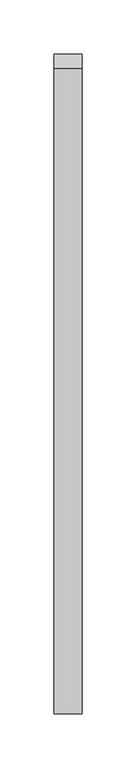
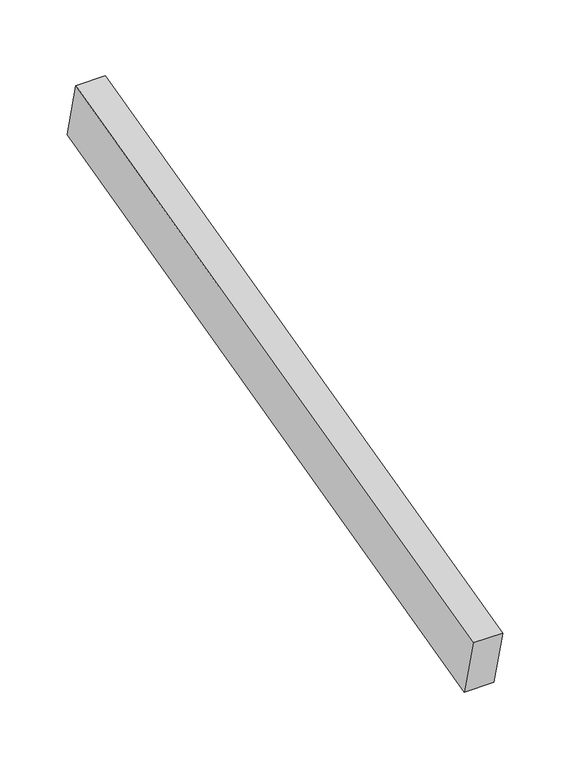
"""IFC4 building model written with IfcOpenShell, lengths in millimetres: proxy geometry, Roof008 1120 : Roof008 1120."""

import ifcopenshell
import ifcopenshell.guid

model = None  # the IFC model being written
_history = None  # IfcOwnerHistory: only IFC2X3 demands one
_inside = {}  # id of a spatial element -> (the spatial element, [elements in it])
_under = {}  # id of a project, library or spatial element -> (it, [spatial elements below it])
_declared = {}  # id of a project -> (the project, [libraries it declares])
_typed = {}  # id of a type object -> (the type object, [elements of that type])
_made_of = {}  # id of a material, layer set ... -> (it, [elements and type objects made of it])


def new_model(schema):
    """Start an empty IFC model of exactly this schema.

    Asked for "IFC4X3", IfcOpenShell would pick the latest addendum, in which some entities
    have other attributes; the version numbers below select the first issue.
    IFC2X3 requires an IfcOwnerHistory on every rooted entity: one is made here for all.
    """
    global model, _history
    if schema == "IFC4X3":
        model = ifcopenshell.file(schema_version=(4, 3, 0, 0))
    else:
        model = ifcopenshell.file(schema=schema)
    _inside.clear()
    _under.clear()
    _declared.clear()
    _typed.clear()
    _made_of.clear()
    _history = None
    if model.schema == "IFC2X3":
        org = make("IfcOrganization", Name="unknown")
        user = make(
            "IfcPersonAndOrganization",
            ThePerson=make("IfcPerson", FamilyName="unknown"),
            TheOrganization=org,
        )
        app = make(
            "IfcApplication",
            ApplicationDeveloper=org,
            Version="unknown",
            ApplicationFullName="unknown",
            ApplicationIdentifier="unknown",
        )
        _history = make(
            "IfcOwnerHistory",
            OwningUser=user,
            OwningApplication=app,
            ChangeAction="ADDED",
            CreationDate=0,
        )
    return model


def make(cls, **values):
    """One entity of the class cls with the attributes given. An attribute that is None is left unset."""
    return model.create_entity(
        cls, **{name: value for name, value in values.items() if value is not None}
    )


def rooted(cls, **values):
    """An entity with a GlobalId (a new one), such as an element, a storey or a relation."""
    return make(cls, GlobalId=ifcopenshell.guid.new(), OwnerHistory=_history, **values)


def si_unit(unit_type, name, prefix=None):
    """IfcSIUnit, for example si_unit("LENGTHUNIT", "METRE", prefix="MILLI")."""
    return make("IfcSIUnit", UnitType=unit_type, Prefix=prefix, Name=name)


def assignment(units):
    """IfcUnitAssignment: the units of a project."""
    return None if units is None else make("IfcUnitAssignment", Units=units)


def point(xyz):
    """IfcCartesianPoint."""
    return None if xyz is None else make("IfcCartesianPoint", Coordinates=xyz)


def direction(xyz):
    """IfcDirection."""
    return None if xyz is None else make("IfcDirection", DirectionRatios=xyz)


def frame(location, z_axis=None, x_axis=None):
    """IfcAxis2Placement3D, a coordinate frame: its origin and axes. An axis left out is left unset."""
    return make(
        "IfcAxis2Placement3D",
        Location=point(location),
        Axis=direction(z_axis),
        RefDirection=direction(x_axis),
    )


def origin():
    """The frame at (0, 0, 0) with its axes left unset."""
    return frame((0.0, 0.0, 0.0))


def place(relative_to, where):
    """IfcLocalPlacement: puts the frame where relative to a parent placement (None: the world)."""
    return make(
        "IfcLocalPlacement", PlacementRelTo=relative_to, RelativePlacement=where
    )


def context(
    kind, dimensions, precision=None, world=None, true_north=None, identifier=None
):
    """IfcGeometricRepresentationContext, for example the 3D "Model" context."""
    return make(
        "IfcGeometricRepresentationContext",
        ContextIdentifier=identifier,
        ContextType=kind,
        CoordinateSpaceDimension=dimensions,
        Precision=precision,
        WorldCoordinateSystem=world,
        TrueNorth=true_north,
    )


def project(units=None, contexts=None):
    """IfcProject with its units and contexts."""
    return rooted(
        "IfcProject",
        Name="project",
        RepresentationContexts=contexts,
        UnitsInContext=assignment(units),
    )


def spatial(cls, under=None, at=None, **own):
    """A site, building, storey or space (cls), placed at a placement, below another one or the project."""
    s = rooted(cls, ObjectPlacement=at, **own)
    if under is not None:
        _under.setdefault(under.id(), (under, []))[1].append(s)
    return s


def polyline(points):
    """IfcPolyline through the points."""
    return make("IfcPolyline", Points=[point(p) for p in points])


def outline(outer, holes=None, kind="AREA"):
    """IfcArbitraryClosedProfileDef: a profile drawn as a closed curve; with holes, ...WithVoids."""
    if holes is None:
        return make("IfcArbitraryClosedProfileDef", ProfileType=kind, OuterCurve=outer)
    return make(
        "IfcArbitraryProfileDefWithVoids",
        ProfileType=kind,
        OuterCurve=outer,
        InnerCurves=holes,
    )


def extrude(swept, where, along, depth):
    """IfcExtrudedAreaSolid: the profile swept, set in the frame where, extruded along a direction by depth."""
    return make(
        "IfcExtrudedAreaSolid",
        SweptArea=swept,
        Position=where,
        ExtrudedDirection=direction(along),
        Depth=depth,
    )


def shape(context_of_items, identifier, shape_type, items):
    """IfcShapeRepresentation: the items that make up one representation, for example the "Body"."""
    return make(
        "IfcShapeRepresentation",
        ContextOfItems=context_of_items,
        RepresentationIdentifier=identifier,
        RepresentationType=shape_type,
        Items=items,
    )


def source(mapping_origin, context_of_items, identifier, shape_type, items):
    """IfcRepresentationMap: a shape defined once, which mapped items show again and again."""
    return make(
        "IfcRepresentationMap",
        MappingOrigin=mapping_origin,
        MappedRepresentation=shape(context_of_items, identifier, shape_type, items),
    )


def transform(
    local_origin,
    x_axis=None,
    y_axis=None,
    z_axis=None,
    scale=None,
    scale2=None,
    scale3=None,
    uniform=True,
):
    """IfcCartesianTransformationOperator3D, or its non-uniform kind. x_axis, y_axis, z_axis: its Axis1, 2, 3."""
    if uniform:
        return make(
            "IfcCartesianTransformationOperator3D",
            Axis1=direction(x_axis),
            Axis2=direction(y_axis),
            LocalOrigin=point(local_origin),
            Scale=scale,
            Axis3=direction(z_axis),
        )
    return make(
        "IfcCartesianTransformationOperator3DnonUniform",
        Axis1=direction(x_axis),
        Axis2=direction(y_axis),
        LocalOrigin=point(local_origin),
        Scale=scale,
        Axis3=direction(z_axis),
        Scale2=scale2,
        Scale3=scale3,
    )


def mapped(mapping_source, mapping_target):
    """IfcMappedItem: shows the shape of a source again, moved by a transform."""
    return make(
        "IfcMappedItem", MappingSource=mapping_source, MappingTarget=mapping_target
    )


def made_of(thing, what):
    """Note that an element or type object is made of a material, layer set ...; save() writes the relation."""
    if what is not None:
        _made_of.setdefault(what.id(), (what, []))[1].append(thing)
    return thing


def element(
    cls,
    number,
    at=None,
    inside=None,
    cuts=None,
    type_object=None,
    material=None,
    context=None,
    identifier="Body",
    shape_type=None,
    held_by="IfcProductDefinitionShape",
    body=None,
    shapes=None,
    **own,
):
    """One element of the class cls, such as IfcWall. Its Tag is "e" and its number.

    at: its placement. inside: the storey or other place that contains it. cuts: it is an
    opening in that element (IfcRelVoidsElement). A single representation is given by context,
    identifier, shape_type and body (its items); several are given by shapes. held_by: the class
    of the entity that holds the representations. save() writes the other relations.
    """
    e = rooted(cls, Tag="e%d" % number, ObjectPlacement=at, **own)
    if body is not None:
        shapes = [shape(context, identifier, shape_type, body)]
    if shapes is not None:
        e.Representation = make(held_by, Representations=shapes)
    if inside is not None:
        _inside.setdefault(inside.id(), (inside, []))[1].append(e)
    if cuts is not None:
        rooted(
            "IfcRelVoidsElement", RelatingBuildingElement=cuts, RelatedOpeningElement=e
        )
    if type_object is not None:
        _typed.setdefault(type_object.id(), (type_object, []))[1].append(e)
    return made_of(e, material)


def aggregate(whole, parts):
    """IfcRelAggregates: a whole, such as a stair, and the parts it consists of."""
    return rooted("IfcRelAggregates", RelatingObject=whole, RelatedObjects=parts)


def save(model, path):
    """Write the relations noted so far, then the file.

    IfcRelAggregates (storeys below a building ...), IfcRelContainedInSpatialStructure (elements
    in a storey), IfcRelDefinesByType, IfcRelAssociatesMaterial and IfcRelDeclares: one each for
    every whole, place, type object, material and project.
    """
    for whole, parts in _under.values():
        aggregate(whole, parts)
    for where, things in _inside.values():
        rooted(
            "IfcRelContainedInSpatialStructure",
            RelatedElements=things,
            RelatingStructure=where,
        )
    for kind, things in _typed.values():
        rooted("IfcRelDefinesByType", RelatedObjects=things, RelatingType=kind)
    for what, things in _made_of.values():
        rooted("IfcRelAssociatesMaterial", RelatedObjects=things, RelatingMaterial=what)
    for by, libraries in _declared.values():
        rooted("IfcRelDeclares", RelatingContext=by, RelatedDefinitions=libraries)
    model.write(path)


def generic_models_6bafc0a9(model_context):
    return source(origin(), model_context, "Body", "SweptSolid", [
        extrude(outline(polyline([(10169.6304502, 43758.3868694), (10156.4176865, 43811.2379242), (10748.8728775, 43959.34982), (10762.0851937, 43906.5005553), (10169.6304502, 43758.3868694)])), frame((4168.9879286, 0.0, 0.0), z_axis=(1.0, 0.0, 0.0), x_axis=(0.0, 1.0, 0.0)), (0.0, 0.0, 1.0), 25.4),
    ])


if __name__ == "__main__":
    model = new_model("IFC4")
    model_context = context("Model", 3, world=origin())
    ifc_project = project(units=[si_unit("LENGTHUNIT", "METRE", prefix="MILLI")], contexts=[model_context])
    site = spatial("IfcSite", under=ifc_project)
    building = spatial("IfcBuilding", under=site)
    placement = place(None, origin())
    generic_models_shape = generic_models_6bafc0a9(model_context)
    element("IfcBuildingElementProxy", 1, Name="Roof008 1120 : Roof008 1120", ObjectType="Roof008 1120 : Roof008 1120", at=placement, inside=building, context=model_context, shape_type="MappedRepresentation", body=[
        mapped(generic_models_shape, transform((0.0, 0.0, 0.0), x_axis=(1.0, 0.0, 0.0), y_axis=(0.0, 1.0, 0.0), z_axis=(0.0, 0.0, 1.0))),
    ])
    save(model, "model.ifc")

# Revit data of these elements
# Type "Roof008 1120 : Roof008 1120"
#   NameOverride = "Roof008"
# Element 1 (IfcBuildingElementProxy, "Roof008 1120 : Roof008 1120")
#   Materials on its faces: "STANDING SEAM METAL ROOF"
# Materials
#   "STANDING SEAM METAL ROOF": class "Unassigned", colour RGB 128 128 128, transparency 0
